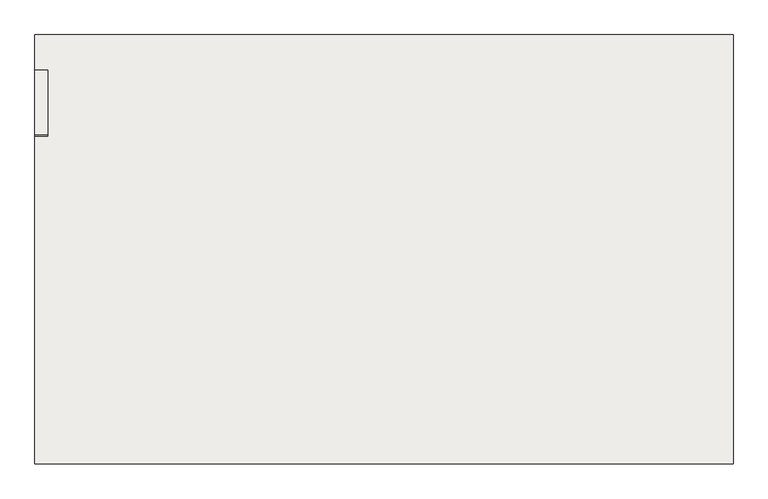
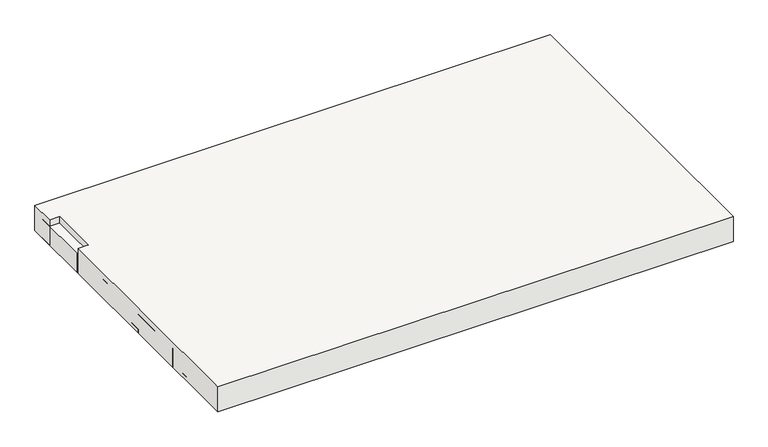
"""IFC4 building model written with IfcOpenShell, lengths in millimetres: slab geometry, Pano 7 (16 cm)."""

from ifc_helpers import new_model, si_unit, origin, origin_with_axes, place, context, project, spatial, polyline, outline, extrude, source, transform, mapped, element, save


def slab_50387449(model_context):
    return source(origin(), model_context, "Body", "SweptSolid", [
        extrude(outline(polyline([(2255.00107, 11155.0), (2255.00107, 10700.06948), (2255.0, 9240.0), (-860.0, 9240.0), (-860.0, 10700.0), (-800.0, 10700.0), (-800.0, 11000.0), (-860.0, 11000.0), (-860.0, 11155.0), (2255.00107, 11155.0)])), origin_with_axes(), (0.0, 0.0, 1.0), 160.0),
        extrude(outline(polyline([(-860.0, 9711.0), (-860.0, 10071.0), (-365.0, 10071.0), (-365.0, 9711.0), (-860.0, 9711.0)])), origin_with_axes(), (0.0, 0.0, 1.0), 120.0),
        extrude(outline(polyline([(640.0, 10211.0), (640.0, 10571.0), (1135.0, 10571.0), (1135.0, 10211.0), (640.0, 10211.0)])), origin_with_axes(), (0.0, 0.0, 1.0), 120.0),
        extrude(outline(polyline([(-860.0, 10071.0), (-860.0, 10211.0), (2255.00107, 10211.0), (2255.00107, 10071.0), (-860.0, 10071.0)])), origin_with_axes(), (0.0, 0.0, 1.0), 24.0),
        extrude(outline(polyline([(1640.0, 9711.0), (1640.0, 10071.0), (2135.0, 10071.0), (2135.0, 9711.0), (1640.0, 9711.0)])), origin_with_axes(), (0.0, 0.0, 1.0), 120.0),
        extrude(outline(polyline([(140.0, 10211.0), (140.0, 10571.0), (635.0, 10571.0), (635.0, 10211.0), (140.0, 10211.0)])), origin_with_axes(), (0.0, 0.0, 1.0), 120.0),
        extrude(outline(polyline([(-860.0, 10211.0), (-860.0, 10571.0), (-365.0, 10571.0), (-365.0, 10211.0), (-860.0, 10211.0)])), origin_with_axes(), (0.0, 0.0, 1.0), 120.0),
        extrude(outline(polyline([(-360.0, 10211.0), (-360.0, 10571.0), (135.0, 10571.0), (135.0, 10211.0), (-360.0, 10211.0)])), origin_with_axes(), (0.0, 0.0, 1.0), 120.0),
        extrude(outline(polyline([(640.0, 9711.0), (640.0, 10071.0), (1135.0, 10071.0), (1135.0, 9711.0), (640.0, 9711.0)])), origin_with_axes(), (0.0, 0.0, 1.0), 120.0),
        extrude(outline(polyline([(1140.0, 9711.0), (1140.0, 10071.0), (1635.0, 10071.0), (1635.0, 9711.0), (1140.0, 9711.0)])), origin_with_axes(), (0.0, 0.0, 1.0), 120.0),
        extrude(outline(polyline([(1140.0, 10211.0), (1140.0, 10571.0), (1635.0, 10571.0), (1635.0, 10211.0), (1140.0, 10211.0)])), origin_with_axes(), (0.0, 0.0, 1.0), 120.0),
        extrude(outline(polyline([(-360.0, 9711.0), (-360.0, 10071.0), (135.0, 10071.0), (135.0, 9711.0), (-360.0, 9711.0)])), origin_with_axes(), (0.0, 0.0, 1.0), 120.0),
        extrude(outline(polyline([(-860.0, 9571.0), (-860.0, 9711.0), (2255.00107, 9711.0), (2255.00107, 9571.0), (-860.0, 9571.0)])), origin_with_axes(), (0.0, 0.0, 1.0), 24.0),
        extrude(outline(polyline([(2140.0, 10710.5), (2140.0, 11070.5), (2250.00107, 11070.5), (2250.00107, 10710.5), (2140.0, 10710.5)])), origin_with_axes(), (0.0, 0.0, 1.0), 120.0),
        extrude(outline(polyline([(-860.0, 10571.0), (-860.0, 10711.0), (2255.00107, 10711.0), (2255.00107, 10571.0), (-860.0, 10571.0)])), origin_with_axes(), (0.0, 0.0, 1.0), 24.0),
        extrude(outline(polyline([(-860.0, 10710.5), (-860.0, 11070.5), (-365.0, 11070.5), (-365.0, 10710.5), (-860.0, 10710.5)])), origin_with_axes(), (0.0, 0.0, 1.0), 120.0),
        extrude(outline(polyline([(1640.0, 10710.5), (1640.0, 11070.5), (2135.0, 11070.5), (2135.0, 10710.5), (1640.0, 10710.5)])), origin_with_axes(), (0.0, 0.0, 1.0), 120.0),
        extrude(outline(polyline([(2140.0, 9711.0), (2140.0, 10071.0), (2250.00107, 10071.0), (2250.00107, 9711.0), (2140.0, 9711.0)])), origin_with_axes(), (0.0, 0.0, 1.0), 120.0),
        extrude(outline(polyline([(140.0, 9711.0), (140.0, 10071.0), (635.0, 10071.0), (635.0, 9711.0), (140.0, 9711.0)])), origin_with_axes(), (0.0, 0.0, 1.0), 120.0),
        extrude(outline(polyline([(140.0, 10710.5), (140.0, 11070.5), (635.0, 11070.5), (635.0, 10710.5), (140.0, 10710.5)])), origin_with_axes(), (0.0, 0.0, 1.0), 120.0),
        extrude(outline(polyline([(-360.0, 10710.5), (-360.0, 11070.5), (135.0, 11070.5), (135.0, 10710.5), (-360.0, 10710.5)])), origin_with_axes(), (0.0, 0.0, 1.0), 120.0),
        extrude(outline(polyline([(2140.0, 10211.0), (2140.0, 10571.0), (2250.00107, 10571.0), (2250.00107, 10211.0), (2140.0, 10211.0)])), origin_with_axes(), (0.0, 0.0, 1.0), 120.0),
        extrude(outline(polyline([(640.0, 10710.5), (640.0, 11070.5), (1135.0, 11070.5), (1135.0, 10710.5), (640.0, 10710.5)])), origin_with_axes(), (0.0, 0.0, 1.0), 120.0),
        extrude(outline(polyline([(1140.0, 10710.5), (1140.0, 11070.5), (1635.0, 11070.5), (1635.0, 10710.5), (1140.0, 10710.5)])), origin_with_axes(), (0.0, 0.0, 1.0), 120.0),
        extrude(outline(polyline([(1640.0, 10211.0), (1640.0, 10571.0), (2135.0, 10571.0), (2135.0, 10211.0), (1640.0, 10211.0)])), origin_with_axes(), (0.0, 0.0, 1.0), 120.0),
    ])


if __name__ == "__main__":
    model = new_model("IFC4")
    model_context = context("Model", 3, world=origin())
    ifc_project = project(units=[si_unit("LENGTHUNIT", "METRE", prefix="MILLI")], contexts=[model_context])
    site = spatial("IfcSite", under=ifc_project)
    building = spatial("IfcBuilding", under=site)
    placement = place(None, origin())
    slab_shape = slab_50387449(model_context)
    element("IfcSlab", 1, ObjectType="Pano 7 (16 cm)", at=placement, inside=building, context=model_context, shape_type="MappedRepresentation", body=[
        mapped(slab_shape, transform((0.0, 0.0, 0.0), x_axis=(1.0, 0.0, 0.0), y_axis=(0.0, 1.0, 0.0), z_axis=(0.0, 0.0, 1.0))),
    ])
    save(model, "model.ifc")

# Revit data of these elements
# Element 1 (IfcSlab, "Pano 7 (16 cm)")
#   Materials on its faces: "Molde de poliestireno", "Concreto armado", "RGB 168-169-158"
# Materials
#   "Molde de poliestireno": class "Não atribuído", colour RGB 255 255 255, transparency 0
#   "Concreto armado": class "Não atribuído", colour RGB 168 169 158, transparency 0
#   "RGB 168-169-158": class "Não atribuído", colour RGB 168 169 158, transparency 0
